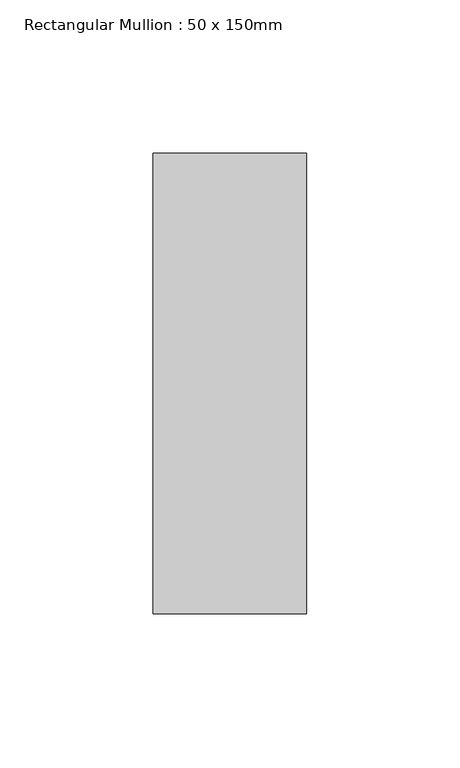
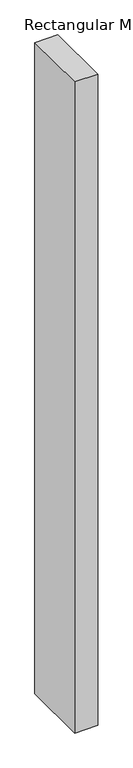
"""IFC4 building model written with IfcOpenShell, lengths in millimetres: member geometry, Rectangular Mullion : 50 x 150mm."""

import ifcopenshell
import ifcopenshell.guid

model = None  # the IFC model being written
_history = None  # IfcOwnerHistory: only IFC2X3 demands one
_inside = {}  # id of a spatial element -> (the spatial element, [elements in it])
_under = {}  # id of a project, library or spatial element -> (it, [spatial elements below it])
_declared = {}  # id of a project -> (the project, [libraries it declares])
_typed = {}  # id of a type object -> (the type object, [elements of that type])
_made_of = {}  # id of a material, layer set ... -> (it, [elements and type objects made of it])


def new_model(schema):
    """Start an empty IFC model of exactly this schema.

    Asked for "IFC4X3", IfcOpenShell would pick the latest addendum, in which some entities
    have other attributes; the version numbers below select the first issue.
    IFC2X3 requires an IfcOwnerHistory on every rooted entity: one is made here for all.
    """
    global model, _history
    if schema == "IFC4X3":
        model = ifcopenshell.file(schema_version=(4, 3, 0, 0))
    else:
        model = ifcopenshell.file(schema=schema)
    _inside.clear()
    _under.clear()
    _declared.clear()
    _typed.clear()
    _made_of.clear()
    _history = None
    if model.schema == "IFC2X3":
        org = make("IfcOrganization", Name="unknown")
        user = make(
            "IfcPersonAndOrganization",
            ThePerson=make("IfcPerson", FamilyName="unknown"),
            TheOrganization=org,
        )
        app = make(
            "IfcApplication",
            ApplicationDeveloper=org,
            Version="unknown",
            ApplicationFullName="unknown",
            ApplicationIdentifier="unknown",
        )
        _history = make(
            "IfcOwnerHistory",
            OwningUser=user,
            OwningApplication=app,
            ChangeAction="ADDED",
            CreationDate=0,
        )
    return model


def make(cls, **values):
    """One entity of the class cls with the attributes given. An attribute that is None is left unset."""
    return model.create_entity(
        cls, **{name: value for name, value in values.items() if value is not None}
    )


def rooted(cls, **values):
    """An entity with a GlobalId (a new one), such as an element, a storey or a relation."""
    return make(cls, GlobalId=ifcopenshell.guid.new(), OwnerHistory=_history, **values)


def si_unit(unit_type, name, prefix=None):
    """IfcSIUnit, for example si_unit("LENGTHUNIT", "METRE", prefix="MILLI")."""
    return make("IfcSIUnit", UnitType=unit_type, Prefix=prefix, Name=name)


def assignment(units):
    """IfcUnitAssignment: the units of a project."""
    return None if units is None else make("IfcUnitAssignment", Units=units)


def point(xyz):
    """IfcCartesianPoint."""
    return None if xyz is None else make("IfcCartesianPoint", Coordinates=xyz)


def direction(xyz):
    """IfcDirection."""
    return None if xyz is None else make("IfcDirection", DirectionRatios=xyz)


def frame(location, z_axis=None, x_axis=None):
    """IfcAxis2Placement3D, a coordinate frame: its origin and axes. An axis left out is left unset."""
    return make(
        "IfcAxis2Placement3D",
        Location=point(location),
        Axis=direction(z_axis),
        RefDirection=direction(x_axis),
    )


def origin():
    """The frame at (0, 0, 0) with its axes left unset."""
    return frame((0.0, 0.0, 0.0))


def place(relative_to, where):
    """IfcLocalPlacement: puts the frame where relative to a parent placement (None: the world)."""
    return make(
        "IfcLocalPlacement", PlacementRelTo=relative_to, RelativePlacement=where
    )


def context(
    kind, dimensions, precision=None, world=None, true_north=None, identifier=None
):
    """IfcGeometricRepresentationContext, for example the 3D "Model" context."""
    return make(
        "IfcGeometricRepresentationContext",
        ContextIdentifier=identifier,
        ContextType=kind,
        CoordinateSpaceDimension=dimensions,
        Precision=precision,
        WorldCoordinateSystem=world,
        TrueNorth=true_north,
    )


def project(units=None, contexts=None):
    """IfcProject with its units and contexts."""
    return rooted(
        "IfcProject",
        Name="project",
        RepresentationContexts=contexts,
        UnitsInContext=assignment(units),
    )


def spatial(cls, under=None, at=None, **own):
    """A site, building, storey or space (cls), placed at a placement, below another one or the project."""
    s = rooted(cls, ObjectPlacement=at, **own)
    if under is not None:
        _under.setdefault(under.id(), (under, []))[1].append(s)
    return s


def polyline(points):
    """IfcPolyline through the points."""
    return make("IfcPolyline", Points=[point(p) for p in points])


def outline(outer, holes=None, kind="AREA"):
    """IfcArbitraryClosedProfileDef: a profile drawn as a closed curve; with holes, ...WithVoids."""
    if holes is None:
        return make("IfcArbitraryClosedProfileDef", ProfileType=kind, OuterCurve=outer)
    return make(
        "IfcArbitraryProfileDefWithVoids",
        ProfileType=kind,
        OuterCurve=outer,
        InnerCurves=holes,
    )


def extrude(swept, where, along, depth):
    """IfcExtrudedAreaSolid: the profile swept, set in the frame where, extruded along a direction by depth."""
    return make(
        "IfcExtrudedAreaSolid",
        SweptArea=swept,
        Position=where,
        ExtrudedDirection=direction(along),
        Depth=depth,
    )


def shape(context_of_items, identifier, shape_type, items):
    """IfcShapeRepresentation: the items that make up one representation, for example the "Body"."""
    return make(
        "IfcShapeRepresentation",
        ContextOfItems=context_of_items,
        RepresentationIdentifier=identifier,
        RepresentationType=shape_type,
        Items=items,
    )


def source(mapping_origin, context_of_items, identifier, shape_type, items):
    """IfcRepresentationMap: a shape defined once, which mapped items show again and again."""
    return make(
        "IfcRepresentationMap",
        MappingOrigin=mapping_origin,
        MappedRepresentation=shape(context_of_items, identifier, shape_type, items),
    )


def transform(
    local_origin,
    x_axis=None,
    y_axis=None,
    z_axis=None,
    scale=None,
    scale2=None,
    scale3=None,
    uniform=True,
):
    """IfcCartesianTransformationOperator3D, or its non-uniform kind. x_axis, y_axis, z_axis: its Axis1, 2, 3."""
    if uniform:
        return make(
            "IfcCartesianTransformationOperator3D",
            Axis1=direction(x_axis),
            Axis2=direction(y_axis),
            LocalOrigin=point(local_origin),
            Scale=scale,
            Axis3=direction(z_axis),
        )
    return make(
        "IfcCartesianTransformationOperator3DnonUniform",
        Axis1=direction(x_axis),
        Axis2=direction(y_axis),
        LocalOrigin=point(local_origin),
        Scale=scale,
        Axis3=direction(z_axis),
        Scale2=scale2,
        Scale3=scale3,
    )


def mapped(mapping_source, mapping_target):
    """IfcMappedItem: shows the shape of a source again, moved by a transform."""
    return make(
        "IfcMappedItem", MappingSource=mapping_source, MappingTarget=mapping_target
    )


def made_of(thing, what):
    """Note that an element or type object is made of a material, layer set ...; save() writes the relation."""
    if what is not None:
        _made_of.setdefault(what.id(), (what, []))[1].append(thing)
    return thing


def element(
    cls,
    number,
    at=None,
    inside=None,
    cuts=None,
    type_object=None,
    material=None,
    context=None,
    identifier="Body",
    shape_type=None,
    held_by="IfcProductDefinitionShape",
    body=None,
    shapes=None,
    **own,
):
    """One element of the class cls, such as IfcWall. Its Tag is "e" and its number.

    at: its placement. inside: the storey or other place that contains it. cuts: it is an
    opening in that element (IfcRelVoidsElement). A single representation is given by context,
    identifier, shape_type and body (its items); several are given by shapes. held_by: the class
    of the entity that holds the representations. save() writes the other relations.
    """
    e = rooted(cls, Tag="e%d" % number, ObjectPlacement=at, **own)
    if body is not None:
        shapes = [shape(context, identifier, shape_type, body)]
    if shapes is not None:
        e.Representation = make(held_by, Representations=shapes)
    if inside is not None:
        _inside.setdefault(inside.id(), (inside, []))[1].append(e)
    if cuts is not None:
        rooted(
            "IfcRelVoidsElement", RelatingBuildingElement=cuts, RelatedOpeningElement=e
        )
    if type_object is not None:
        _typed.setdefault(type_object.id(), (type_object, []))[1].append(e)
    return made_of(e, material)


def aggregate(whole, parts):
    """IfcRelAggregates: a whole, such as a stair, and the parts it consists of."""
    return rooted("IfcRelAggregates", RelatingObject=whole, RelatedObjects=parts)


def save(model, path):
    """Write the relations noted so far, then the file.

    IfcRelAggregates (storeys below a building ...), IfcRelContainedInSpatialStructure (elements
    in a storey), IfcRelDefinesByType, IfcRelAssociatesMaterial and IfcRelDeclares: one each for
    every whole, place, type object, material and project.
    """
    for whole, parts in _under.values():
        aggregate(whole, parts)
    for where, things in _inside.values():
        rooted(
            "IfcRelContainedInSpatialStructure",
            RelatedElements=things,
            RelatingStructure=where,
        )
    for kind, things in _typed.values():
        rooted("IfcRelDefinesByType", RelatedObjects=things, RelatingType=kind)
    for what, things in _made_of.values():
        rooted("IfcRelAssociatesMaterial", RelatedObjects=things, RelatingMaterial=what)
    for by, libraries in _declared.values():
        rooted("IfcRelDeclares", RelatingContext=by, RelatedDefinitions=libraries)
    model.write(path)


def rectangular_mullion_50_x_150mm_461a195c(model_context):
    return source(origin(), model_context, "Body", "SweptSolid", [
        extrude(outline(polyline([(0.0, 75.0), (0.0, -75.0), (-50.0, -75.0), (-50.0, 75.0), (0.0, 75.0)])), frame((0.0, 0.0, -1500.0), z_axis=(0.0, 0.0, 1.0), x_axis=(1.0, 0.0, 0.0)), (0.0, 0.0, 1.0), 1500.0),
    ])


if __name__ == "__main__":
    model = new_model("IFC4")
    model_context = context("Model", 3, world=origin())
    ifc_project = project(units=[si_unit("LENGTHUNIT", "METRE", prefix="MILLI")], contexts=[model_context])
    site = spatial("IfcSite", under=ifc_project)
    building = spatial("IfcBuilding", under=site)
    placement = place(None, origin())
    rectangular_mullion_50_x_150mm_shape = rectangular_mullion_50_x_150mm_461a195c(model_context)
    element("IfcMember", 1, ObjectType="Rectangular Mullion : 50 x 150mm", at=placement, inside=building, context=model_context, shape_type="MappedRepresentation", body=[
        mapped(rectangular_mullion_50_x_150mm_shape, transform((0.0, 0.0, 0.0), x_axis=(1.0, 0.0, 0.0), y_axis=(0.0, 1.0, 0.0), z_axis=(0.0, 0.0, 1.0))),
    ])
    save(model, "model.ifc")

# Revit data of these elements
# Type "Rectangular Mullion : 50 x 150mm"
#   built-in parameter 1007304 = 0.492126 (stored number, unit not read)
#   built-in parameter 1007301 = 0.082021 (stored number, unit not read)
#   built-in parameter 1007300 = 0.082021 (stored number, unit not read)
# Element 1 (IfcMember, "Rectangular Mullion : 50 x 150mm")
#   Materials on its faces: "Metal - Aluminium"
# Materials
#   "Metal - Aluminium": class "Metal", colour RGB 247 247 247, transparency 0
